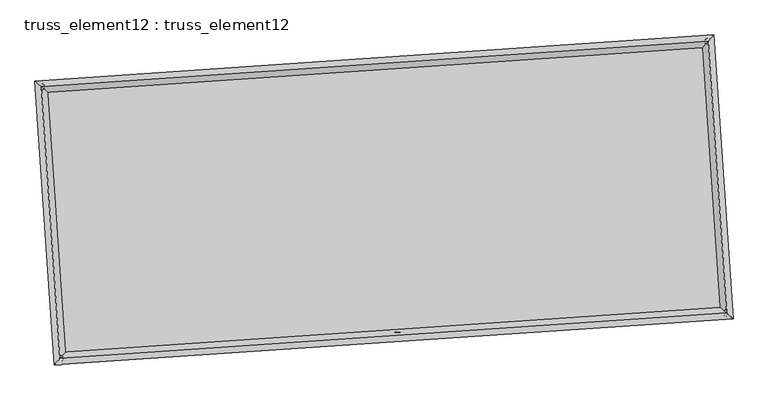
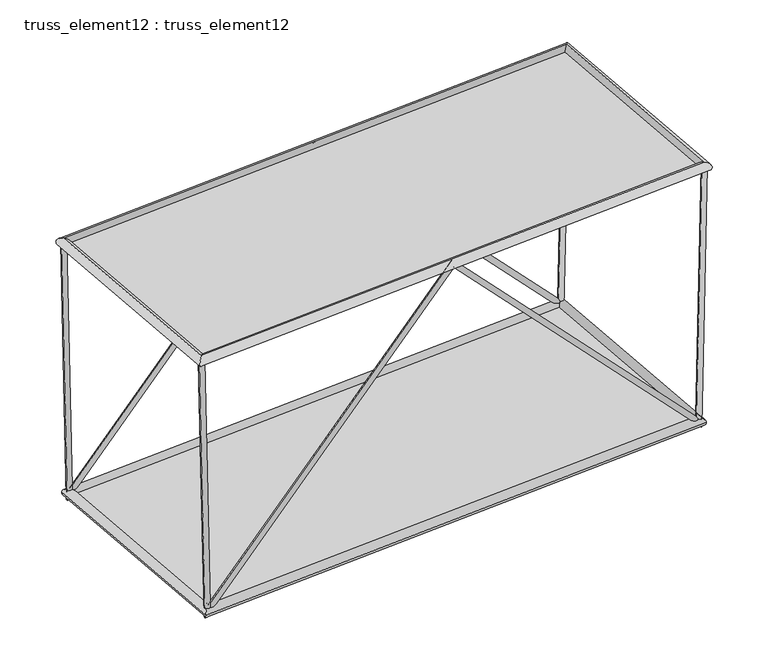
"""IFC4 building model written with IfcOpenShell, lengths in millimetres: plate geometry, truss_element12 : truss_element12."""

from ifc_helpers import new_model, si_unit, frame, origin, origin_with_axes, place, context, project, spatial, polyline, circle_curve, ellipse_curve, outline, extrude, source, transform, mapped, element, save
from ifc_brep_helpers import plane_surface, cylinder_surface, advanced_brep


def truss_element12_truss_element12_2eb2766b(model_context):
    return source(origin(), model_context, "Body", "SolidModel", [
        advanced_brep(
        [(-3777.0986173, 2268.576399, 4999.8579637), (-3876.1768274, 2255.2168966, 4997.6147546), (-3667.6514402, 2276.039186, 121.3427216), (-3761.3354427, 2263.0474941, -121.3427216), (1064.1379984, 2598.6819206, 5070.8413429), (1064.5799486, 2592.1083196, 4926.6125785), (5795.1101519, 2921.2689276, 121.3370387), (5889.6508251, 2921.1115609, -121.3370387), (5905.3685517, 2928.7870288, 4999.8474769), (6005.3427871, 2929.000156, 4997.5876475)],
        [
            (0, 1, circle_curve(frame((-3826.6377224, 2261.8966478, 4998.7363592), z_axis=(-0.022428856188338092, -0.001529338443418397, 0.9997472718312407), x_axis=(-0.1335955670889367, 0.9910348281827929, -0.0014811424265438755)), 50.0)),
            (1, 0, circle_curve(frame((-3826.6377224, 2261.8966478, 4998.7363592), z_axis=(-0.022428856188338092, -0.001529338443418397, 0.9997472718312407), x_axis=(-0.1335955670889367, 0.9910348281827929, -0.0014811424265438755)), 50.0)),
            (0, 2),
            (2, 3, ellipse_curve(frame((-3714.4934414, 2269.54334, 0.0), z_axis=(-0.9298803947541627, -0.06340500931197944, 0.3623565319488393), x_axis=(0.36151709538463256, 0.0246504764791416, 0.9320395612601483)), 130.4740125, 50.0)),
            (3, 1),
            (3, 2, ellipse_curve(frame((-3714.4934414, 2269.54334, 0.0), z_axis=(-0.9298803947541627, -0.06340500931197944, 0.3623565319488393), x_axis=(0.36151709538463256, 0.0246504764791416, 0.9320395612601483)), 130.4740125, 50.0)),
            (2, 4),
            (4, 5, ellipse_curve(frame((1064.3589735, 2595.3951201, 4998.7269607), z_axis=(-0.9976833951339081, -0.06802823816454029, 4.343163055355918e-05), x_axis=(-4.333101666782894e-05, -2.954577309750225e-06, -0.9999999990568467)), 72.2714089, 50.0)),
            (5, 3),
            (5, 4, ellipse_curve(frame((1064.3589735, 2595.3951201, 4998.7269607), z_axis=(-0.9976833951339081, -0.06802823816454029, 4.343163055355918e-05), x_axis=(-4.333101666782894e-05, -2.954577309750225e-06, -0.9999999990568467)), 72.2714089, 50.0)),
            (4, 6),
            (6, 7, ellipse_curve(frame((5842.3804885, 2921.1902443, 0.0), z_axis=(-0.9299262044326752, -0.06340813289981873, -0.3622384062901084), x_axis=(-0.3613992433762661, -0.02464244059868868, 0.9320854773079572)), 130.4614748, 50.0)),
            (7, 5),
            (7, 6, ellipse_curve(frame((5842.3804885, 2921.1902443, 0.0), z_axis=(-0.9299262044326752, -0.06340813289981873, -0.3622384062901084), x_axis=(-0.3613992433762661, -0.02464244059868868, 0.9320854773079572)), 130.4614748, 50.0)),
            (8, 9, circle_curve(frame((5955.3556694, 2928.8935924, 4998.7175622), z_axis=(0.02259503617534383, 0.0015406696250230578, 0.9997435124457381), x_axis=(-0.0021655416851002326, 0.9999965420027805, -0.0014921165139930713)), 50.0)),
            (9, 8, circle_curve(frame((5955.3556694, 2928.8935924, 4998.7175622), z_axis=(0.02259503617534383, 0.0015406696250230578, 0.9997435124457381), x_axis=(-0.0021655416851002326, 0.9999965420027805, -0.0014921165139930713)), 50.0)),
            (6, 8),
            (9, 7),
        ],
        [
            plane_surface(frame((-3826.6377224, 2311.8965893, 4998.8128453), z_axis=(-0.022428856188340066, -0.0015293384434182614, 0.9997472718312406), x_axis=(0.9997484415642182, -3.430994296671485e-05, 0.02242882994596584))),
            cylinder_surface(frame((-3826.6377224, 2261.8966478, 4998.7363592), z_axis=(-0.022428856188338092, -0.001529338443418397, 0.9997472718312407), x_axis=(-0.1335955670889367, 0.9910348281827929, -0.0014811424265438755)), 50.0),
            cylinder_surface(frame((-3714.4934414, 2269.54334, 0.0), z_axis=(-0.6902650946631375, -0.04706655286180253, -0.722024126114493), x_axis=(-0.020420522547065688, 0.9987518042514819, -0.045583283814512085)), 50.0),
            cylinder_surface(frame((1064.3589735, 2595.3951201, 4998.7269607), z_axis=(-0.6902025199802069, -0.04706228613204244, 0.7220842212907008), x_axis=(-0.11534428927699865, 0.9922793134371867, -0.0455791515477154)), 50.0),
            plane_surface(frame((5955.3556694, 2878.8936517, 4998.7946154), z_axis=(0.02259503617534488, 0.0015406696250278675, 0.999743512445738), x_axis=(0.9997446995809655, -3.482037556779006e-05, -0.022595009345131704))),
            cylinder_surface(frame((5842.3804885, 2921.1902443, 0.0), z_axis=(-0.022595036175343825, -0.0015406696250230573, -0.9997435124457379), x_axis=(-0.0021655416851002326, 0.9999965420027805, -0.0014921165139930713)), 50.0),
        ],
        [
            (0, [[1, 2]]),
            (1, [[-1, 3, 4, 5]]),
            (1, [[-2, -5, 6, -3]]),
            (2, [[-4, 7, 8, 9]]),
            (2, [[-6, -9, 10, -7]]),
            (3, [[-8, 11, 12, 13]]),
            (3, [[-10, -13, 14, -11]]),
            (4, [[15, 16]]),
            (5, [[-12, 17, -16, 18]]),
            (5, [[-14, -18, -15, -17]]),
        ],
    ),
        advanced_brep(
        [(-3504.9856644, -1722.1571853, 4999.8579637), (-3604.0638745, -1735.5166877, 4997.6147546), (-3395.5384873, -1714.6943983, 121.3427216), (-3489.2224898, -1727.6860902, -121.3427216), (1336.2509513, -1392.0516637, 5070.8413429), (1336.6929015, -1398.6252647, 4926.6125785), (6067.2231048, -1069.4646567, 121.3370387), (6161.763778, -1069.6220234, -121.3370387), (6177.4815046, -1061.9465555, 4999.8474769), (6277.45574, -1061.7334283, 4997.5876475)],
        [
            (0, 1, circle_curve(frame((-3554.5247694, -1728.8369365, 4998.7363592), z_axis=(-0.022428856188338314, -0.001529338443418425, 0.9997472718312406), x_axis=(-0.13359556708893713, 0.9910348281827928, -0.0014811424265438883)), 50.0)),
            (1, 0, circle_curve(frame((-3554.5247694, -1728.8369365, 4998.7363592), z_axis=(-0.022428856188338314, -0.001529338443418425, 0.9997472718312406), x_axis=(-0.13359556708893713, 0.9910348281827928, -0.0014811424265438883)), 50.0)),
            (0, 2),
            (2, 3, ellipse_curve(frame((-3442.3804885, -1721.1902443, 0.0), z_axis=(-0.9298803947541627, -0.06340500931197972, 0.36235653194883954), x_axis=(0.3615170953846327, 0.024650476479141713, 0.9320395612601483)), 130.4740125, 50.0)),
            (3, 1),
            (3, 2, ellipse_curve(frame((-3442.3804885, -1721.1902443, 0.0), z_axis=(-0.9298803947541627, -0.06340500931197972, 0.36235653194883954), x_axis=(0.3615170953846327, 0.024650476479141713, 0.9320395612601483)), 130.4740125, 50.0)),
            (2, 4),
            (4, 5, ellipse_curve(frame((1336.4719264, -1395.3384642, 4998.7269607), z_axis=(-0.9976833951339081, -0.0680282381645403, 4.343163055428133e-05), x_axis=(-4.333101666844397e-05, -2.954577310067353e-06, -0.9999999990568467)), 72.2714089, 50.0)),
            (5, 3),
            (5, 4, ellipse_curve(frame((1336.4719264, -1395.3384642, 4998.7269607), z_axis=(-0.9976833951339081, -0.0680282381645403, 4.343163055428133e-05), x_axis=(-4.333101666844397e-05, -2.954577310067353e-06, -0.9999999990568467)), 72.2714089, 50.0)),
            (4, 6),
            (6, 7, ellipse_curve(frame((6114.4934414, -1069.54334, 0.0), z_axis=(-0.9299262044326754, -0.06340813289981846, -0.3622384062901074), x_axis=(-0.36139924337626533, -0.024642440598688524, 0.9320854773079577)), 130.4614748, 50.0)),
            (7, 5),
            (7, 6, ellipse_curve(frame((6114.4934414, -1069.54334, 0.0), z_axis=(-0.9299262044326754, -0.06340813289981846, -0.3622384062901074), x_axis=(-0.36139924337626533, -0.024642440598688524, 0.9320854773079577)), 130.4614748, 50.0)),
            (8, 9, circle_curve(frame((6227.4686223, -1061.8399919, 4998.7175622), z_axis=(0.022595036175344883, 0.0015406696250231194, 0.999743512445738), x_axis=(-0.002165541685099796, 0.9999965420027807, -0.001492116513993141)), 50.0)),
            (9, 8, circle_curve(frame((6227.4686223, -1061.8399919, 4998.7175622), z_axis=(0.022595036175344883, 0.0015406696250231194, 0.999743512445738), x_axis=(-0.002165541685099796, 0.9999965420027807, -0.001492116513993141)), 50.0)),
            (6, 8),
            (9, 7),
        ],
        [
            plane_surface(frame((-3554.5247694, -1678.836995, 4998.8128453), z_axis=(-0.022428856188340066, -0.0015293384434182738, 0.9997472718312406), x_axis=(0.9997484415642182, -3.430994296671485e-05, 0.02242882994596584))),
            cylinder_surface(frame((-3554.5247694, -1728.8369365, 4998.7363592), z_axis=(-0.022428856188338314, -0.001529338443418425, 0.9997472718312406), x_axis=(-0.13359556708893713, 0.9910348281827928, -0.0014811424265438883)), 50.0),
            cylinder_surface(frame((-3442.3804885, -1721.1902443, 0.0), z_axis=(-0.6902650946631377, -0.04706655286180275, -0.7220241261144925), x_axis=(-0.020420522547065896, 0.9987518042514819, -0.0455832838145122)), 50.0),
            cylinder_surface(frame((1336.4719264, -1395.3384642, 4998.7269607), z_axis=(-0.6902025199802064, -0.04706228613204221, 0.7220842212907015), x_axis=(-0.11534428927699848, 0.9922793134371867, -0.04557915154771544)), 50.0),
            plane_surface(frame((6227.4686223, -1111.8399326, 4998.7946154), z_axis=(0.022595036175344883, 0.0015406696250278823, 0.999743512445738), x_axis=(0.9997446995809655, -3.482037556823415e-05, -0.022595009345131704))),
            cylinder_surface(frame((6114.4934414, -1069.54334, 0.0), z_axis=(-0.022595036175344883, -0.0015406696250231194, -0.999743512445738), x_axis=(-0.002165541685099796, 0.9999965420027807, -0.001492116513993141)), 50.0),
        ],
        [
            (0, [[1, 2]]),
            (1, [[-1, 3, 4, 5]]),
            (1, [[-2, -5, 6, -3]]),
            (2, [[-4, 7, 8, 9]]),
            (2, [[-6, -9, 10, -7]]),
            (3, [[-8, 11, 12, 13]]),
            (3, [[-10, -13, 14, -11]]),
            (4, [[15, 16]]),
            (5, [[-12, 17, -16, 18]]),
            (5, [[-14, -18, -15, -17]]),
        ],
    ),
        advanced_brep(
        [(-3554.5296519, -1728.8423479, 4908.7363593), (-3554.5198869, -1728.831525, 5088.736359), (-3826.6321505, 2261.8919492, 5088.736359), (-3826.6432942, 2261.9013465, 4908.7363593), (5955.3511312, 2928.8882044, 5088.7175621), (5955.3602076, 2928.8989804, 4908.7175624), (6227.4633947, -1061.8352698, 5088.7175621), (6227.4738499, -1061.844714, 4908.7175624)],
        [
            (0, 1, ellipse_curve(frame((-3554.5247694, -1728.8369365, 4998.7363592), z_axis=(-0.7535719234041577, 0.6573654662781736, 1.3556177561502808e-06), x_axis=(-0.6573654662767888, -0.7535719234053656, 1.355617756150545e-06)), 127.2792206, 90.0)),
            (1, 2),
            (2, 3, ellipse_curve(frame((-3826.6377224, 2261.8966478, 4998.7363592), z_axis=(-0.6573654662767887, -0.7535719234053656, 1.3556177561507926e-06), x_axis=(0.7535719234041576, -0.6573654662781738, -1.3556177561505282e-06)), 127.2792206, 90.0)),
            (3, 0),
            (1, 0, ellipse_curve(frame((-3554.5247694, -1728.8369365, 4998.7363592), z_axis=(-0.7535719234041577, 0.6573654662781736, 1.3556177561502808e-06), x_axis=(-0.6573654662767888, -0.7535719234053656, 1.355617756150545e-06)), 127.2792206, 90.0)),
            (3, 2, ellipse_curve(frame((-3826.6377224, 2261.8966478, 4998.7363592), z_axis=(-0.6573654662767887, -0.7535719234053656, 1.3556177561507926e-06), x_axis=(0.7535719234041576, -0.6573654662781738, -1.3556177561505282e-06)), 127.2792206, 90.0)),
            (2, 4),
            (4, 5, ellipse_curve(frame((5955.3556694, 2928.8935924, 4998.7175622), z_axis=(-0.7535719234041577, 0.6573654662781736, 1.3556177561507757e-06), x_axis=(-0.6573654662767887, -0.7535719234053658, 1.3556177561505453e-06)), 127.2792206, 90.0)),
            (5, 3),
            (5, 4, ellipse_curve(frame((5955.3556694, 2928.8935924, 4998.7175622), z_axis=(-0.7535719234041577, 0.6573654662781736, 1.3556177561507757e-06), x_axis=(-0.6573654662767887, -0.7535719234053658, 1.3556177561505453e-06)), 127.2792206, 90.0)),
            (4, 6),
            (6, 7, ellipse_curve(frame((6227.4686223, -1061.8399919, 4998.7175622), z_axis=(0.6573654662767887, 0.7535719234053656, -1.3556177561502976e-06), x_axis=(-0.7535719234041576, 0.6573654662781738, 1.3556177561505277e-06)), 127.2792206, 90.0)),
            (7, 5),
            (7, 6, ellipse_curve(frame((6227.4686223, -1061.8399919, 4998.7175622), z_axis=(0.6573654662767887, 0.7535719234053656, -1.3556177561502976e-06), x_axis=(-0.7535719234041576, 0.6573654662781738, 1.3556177561505277e-06)), 127.2792206, 90.0)),
            (6, 1),
            (0, 7),
        ],
        [
            cylinder_surface(frame((-3554.5247694, -1728.8369365, 4998.7363592), z_axis=(0.06802823822869572, -0.997683396074877, 0.0), x_axis=(-0.9976833943843263, -0.0680282381134235, 5.821470724249889e-05)), 90.0),
            cylinder_surface(frame((-3826.6377224, 2261.8966478, 4998.7363592), z_axis=(-0.9976833960730437, -0.06802823822857018, 1.9171330161420476e-06), x_axis=(-0.06802823801321035, 0.997683394501182, 5.6297574229395106e-05)), 90.0),
            cylinder_surface(frame((5955.3556694, 2928.8935924, 4998.7175622), z_axis=(-0.06802823822869565, 0.9976833960748769, 0.0), x_axis=(0.9976833945996861, 0.068028238128108, 5.438044121629132e-05)), 90.0),
            cylinder_surface(frame((6227.4686223, -1061.8399919, 4998.7175622), z_axis=(0.9976833960730437, 0.06802823822857008, -1.9171330161416973e-06), x_axis=(0.06802823822857008, -0.9976833944864976, 5.6297574229395106e-05)), 90.0),
        ],
        [
            (0, [[1, 2, 3, 4]]),
            (0, [[5, -4, 6, -2]]),
            (1, [[-3, 7, 8, 9]]),
            (1, [[-6, -9, 10, -7]]),
            (2, [[-8, 11, 12, 13]]),
            (2, [[-10, -13, 14, -11]]),
            (3, [[-12, 15, -1, 16]]),
            (3, [[-14, -16, -5, -15]]),
        ],
    ),
        advanced_brep(
        [(-3358.7115243, -1625.2761972, 0.0), (-3526.0494527, -1817.1042913, 0.0), (-3810.4074885, 2353.2123043, 0.0), (-3618.5793943, 2185.8743758, 0.0), (5926.0494527, 3017.1042913, 0.0), (5758.7115243, 2825.2761972, 0.0), (6210.4074885, -1153.2123043, 0.0), (6018.5793943, -985.8743758, 0.0)],
        [
            (0, 1, ellipse_curve(frame((-3442.3804885, -1721.1902443, 0.0), z_axis=(-0.7535719234054581, 0.6573654662780807, 0.0), x_axis=(-0.6573654662780807, -0.753571923405458, 0.0)), 127.2792206, 90.0)),
            (1, 2),
            (2, 3, ellipse_curve(frame((-3714.4934414, 2269.54334, 0.0), z_axis=(-0.6573654662780807, -0.7535719234054581, 0.0), x_axis=(0.7535719234054581, -0.6573654662780806, 0.0)), 127.2792206, 90.0)),
            (3, 0),
            (1, 0, ellipse_curve(frame((-3442.3804885, -1721.1902443, 0.0), z_axis=(-0.7535719234054581, 0.6573654662780807, 0.0), x_axis=(-0.6573654662780807, -0.753571923405458, 0.0)), 127.2792206, 90.0)),
            (3, 2, ellipse_curve(frame((-3714.4934414, 2269.54334, 0.0), z_axis=(-0.6573654662780807, -0.7535719234054581, 0.0), x_axis=(0.7535719234054581, -0.6573654662780806, 0.0)), 127.2792206, 90.0)),
            (2, 4),
            (4, 5, ellipse_curve(frame((5842.3804885, 2921.1902443, 0.0), z_axis=(-0.7535719234054578, 0.6573654662780809, 0.0), x_axis=(-0.657365466278081, -0.7535719234054578, 0.0)), 127.2792206, 90.0)),
            (5, 3),
            (5, 4, ellipse_curve(frame((5842.3804885, 2921.1902443, 0.0), z_axis=(-0.7535719234054578, 0.6573654662780809, 0.0), x_axis=(-0.657365466278081, -0.7535719234054578, 0.0)), 127.2792206, 90.0)),
            (4, 6),
            (6, 7, ellipse_curve(frame((6114.4934414, -1069.54334, 0.0), z_axis=(0.657365466278081, 0.7535719234054578, 0.0), x_axis=(-0.7535719234054576, 0.6573654662780811, 0.0)), 127.2792206, 90.0)),
            (7, 5),
            (7, 6, ellipse_curve(frame((6114.4934414, -1069.54334, 0.0), z_axis=(0.657365466278081, 0.7535719234054578, 0.0), x_axis=(-0.7535719234054576, 0.6573654662780811, 0.0)), 127.2792206, 90.0)),
            (6, 1),
            (0, 7),
        ],
        [
            cylinder_surface(frame((-3442.3804885, -1721.1902443, 0.0), z_axis=(0.0680282382287018, -0.9976833960748765, 0.0), x_axis=(-0.9976833960748765, -0.0680282382287018, 0.0)), 90.0),
            cylinder_surface(frame((-3714.4934414, 2269.54334, 0.0), z_axis=(-0.9976833960748765, -0.06802823822870124, 0.0), x_axis=(-0.06802823822870124, 0.9976833960748765, 0.0)), 90.0),
            cylinder_surface(frame((5842.3804885, 2921.1902443, 0.0), z_axis=(-0.06802823822870085, 0.9976833960748768, 0.0), x_axis=(0.9976833960748768, 0.06802823822870085, 0.0)), 90.0),
            cylinder_surface(frame((6114.4934414, -1069.54334, 0.0), z_axis=(0.9976833960748767, 0.06802823822870092, 0.0), x_axis=(0.06802823822870092, -0.9976833960748767, 0.0)), 90.0),
        ],
        [
            (0, [[1, 2, 3, 4]]),
            (0, [[5, -4, 6, -2]]),
            (1, [[-3, 7, 8, 9]]),
            (1, [[-6, -9, 10, -7]]),
            (2, [[-8, 11, 12, 13]]),
            (2, [[-10, -13, 14, -11]]),
            (3, [[-12, 15, -1, 16]]),
            (3, [[-14, -16, -5, -15]]),
        ],
    ),
        extrude(outline(polyline([(-3442.3804885, -1721.1902443), (-3714.4934414, 2269.54334), (5842.3804885, 2921.1902443), (6114.4934414, -1069.54334), (-3442.3804885, -1721.1902443)])), origin_with_axes(), (0.0, 0.0, 1.0), 20.0),
        extrude(outline(polyline([(-2000.0000001, 4902.3535072), (1999.9999999, 4902.3535073), (2000.0, -4902.3535072), (-2000.0, -4902.3535072), (-2000.0000001, 4902.3535072)])), frame((1200.41545, 600.028328, 4998.7269607), z_axis=(1.9126917782716947e-06, 1.3041918153820904e-07, 0.9999999999981622), x_axis=(-0.06802823822870187, 0.9976833960748765, 0.0)), (0.0, 0.0, 1.0), 20.0),
    ])


if __name__ == "__main__":
    model = new_model("IFC4")
    model_context = context("Model", 3, world=origin())
    ifc_project = project(units=[si_unit("LENGTHUNIT", "METRE", prefix="MILLI")], contexts=[model_context])
    site = spatial("IfcSite", under=ifc_project)
    building = spatial("IfcBuilding", under=site)
    placement = place(None, origin())
    truss_element12_truss_element12_shape = truss_element12_truss_element12_2eb2766b(model_context)
    element("IfcPlate", 1, ObjectType="truss_element12 : truss_element12", at=placement, inside=building, context=model_context, shape_type="MappedRepresentation", body=[
        mapped(truss_element12_truss_element12_shape, transform((0.0, 0.0, 0.0), x_axis=(1.0, 0.0, 0.0), y_axis=(0.0, 1.0, 0.0), z_axis=(0.0, 0.0, 1.0))),
    ])
    save(model, "model.ifc")

# Revit data of these elements
# Type "truss_element12 : truss_element12"
#   steellbar1 = 90 mm
#   steelbar2 = 50 mm
#   offset1 = 5000 mm
#   M = Default Roof
# Element 1 (IfcPlate, "truss_element12 : truss_element12")
#   Materials on its faces: "Default Roof"
# Materials
#   "Default Roof": class "Miscellaneous", colour RGB 0 127 0, transparency 0, Comments = "Rendering appearance not upgraded Rendering appearance not upgraded ", Cost = 0
